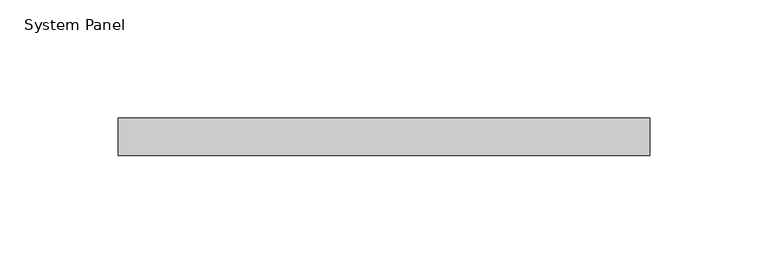
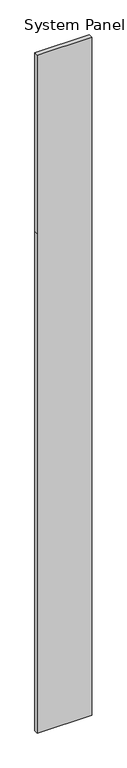
"""IFC4 building model written with IfcOpenShell, lengths in millimetres: plate geometry, System Panel : 로이복층유리_16."""

from ifc_helpers import new_model, si_unit, frame, origin, place, context, project, spatial, polyline, outline, extrude, source, transform, mapped, element, save


def system_panel_845065ac(model_context):
    return source(origin(), model_context, "Body", "SweptSolid", [
        extrude(outline(polyline([(0.0, -112.5000001), (0.0, 112.5000001), (2177.5, 112.5000001), (2955.0, 112.5000001), (2955.0, -112.5000001), (2177.5, -112.5000001), (0.0, -112.5000001)])), frame((0.0, -8.0, 0.0), z_axis=(0.0, 1.0, 0.0), x_axis=(0.0, 0.0, 1.0)), (0.0, 0.0, 1.0), 16.0),
    ])


if __name__ == "__main__":
    model = new_model("IFC4")
    model_context = context("Model", 3, world=origin())
    ifc_project = project(units=[si_unit("LENGTHUNIT", "METRE", prefix="MILLI")], contexts=[model_context])
    site = spatial("IfcSite", under=ifc_project)
    building = spatial("IfcBuilding", under=site)
    placement = place(None, origin())
    system_panel_shape = system_panel_845065ac(model_context)
    element("IfcPlate", 1, ObjectType="System Panel : 로이복층유리_16", at=placement, inside=building, context=model_context, shape_type="MappedRepresentation", body=[
        mapped(system_panel_shape, transform((0.0, 0.0, 0.0), x_axis=(1.0, 0.0, 0.0), y_axis=(0.0, 1.0, 0.0), z_axis=(0.0, 0.0, 1.0))),
    ])
    save(model, "model.ifc")

# Revit data of these elements
# Element 1 (IfcPlate, "System Panel : 로이복층유리_16")
#   Materials on its faces: "00_Glass_Glass"
# Materials
#   "00_Glass_Glass": class "Glass", colour RGB 218 227 224, transparency 0.85, Description = "Glass", Cost = 0, Image = none
